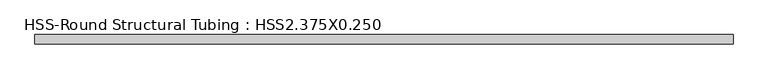
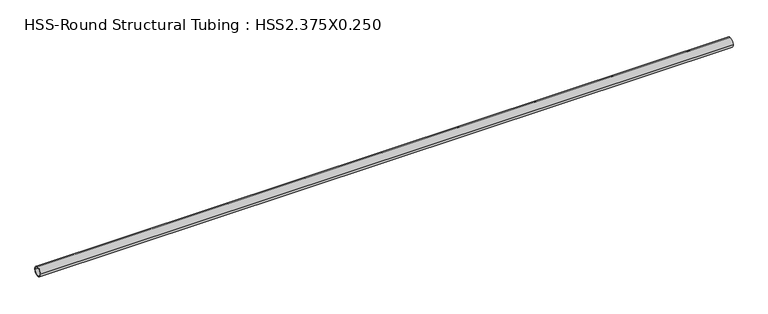
"""IFC4 building model written with IfcOpenShell, lengths in millimetres: beam geometry, HSS-Round Structural Tubing : HSS2.375X0.250."""

from ifc_helpers import new_model, si_unit, point, frame, origin, origin_2d, place, context, project, spatial, circle_curve, trimmed, segment, composite_curve, outline, extrude, source, transform, mapped, element, save


def hss_round_structural_tubing_hss2_375x0_250_6ea9b365(model_context):
    return source(origin(), model_context, "Body", "SweptSolid", [
        extrude(outline(composite_curve([segment(trimmed(circle_curve(origin_2d(), 30.1625), [point((-30.1625, 0.0))], [point((30.1625, 0.0))], False, "CARTESIAN"), True, "CONTINUOUS"), segment(trimmed(circle_curve(origin_2d(), 30.1625), [point((30.1625, 0.0))], [point((-30.1625, 0.0))], False, "CARTESIAN"), True, "CONTINUOUS")], self_intersect=False), holes=[composite_curve([segment(trimmed(circle_curve(origin_2d(), 24.2443), [point((24.2443, 0.0))], [point((-24.2443, 0.0))], True, "CARTESIAN"), True, "CONTINUOUS"), segment(trimmed(circle_curve(origin_2d(), 24.2443), [point((-24.2443, 0.0))], [point((24.2443, 0.0))], True, "CARTESIAN"), True, "CONTINUOUS")], self_intersect=False)]), frame((-2207.2112982, 0.0, 0.0), z_axis=(1.0, 0.0, 0.0), x_axis=(0.0, 1.0, 0.0)), (0.0, 0.0, 1.0), 4401.1362982),
    ])


if __name__ == "__main__":
    model = new_model("IFC4")
    model_context = context("Model", 3, world=origin())
    ifc_project = project(units=[si_unit("LENGTHUNIT", "METRE", prefix="MILLI")], contexts=[model_context])
    site = spatial("IfcSite", under=ifc_project)
    building = spatial("IfcBuilding", under=site)
    placement = place(None, origin())
    hss_round_structural_tubing_hss2_375x0_250_shape = hss_round_structural_tubing_hss2_375x0_250_6ea9b365(model_context)
    element("IfcBeam", 1, ObjectType="HSS-Round Structural Tubing : HSS2.375X0.250", at=placement, inside=building, context=model_context, shape_type="MappedRepresentation", body=[
        mapped(hss_round_structural_tubing_hss2_375x0_250_shape, transform((0.0, 0.0, 0.0), x_axis=(1.0, 0.0, 0.0), y_axis=(0.0, 1.0, 0.0), z_axis=(0.0, 0.0, 1.0))),
    ])
    save(model, "model.ifc")

# Revit data of these elements
# Type "HSS-Round Structural Tubing : HSS2.375X0.250"
#   Assembly Code = "B10"
#   t = 0' - 0.233"
#   W = 5.68
#   Length [instance default] = 5' - 0"
#   OD = 0' - 2 3/8"
#   A = 0.0109028 SF
#   Structural Material [instance default] = Steel ASTM A500, Grade B, Round
# Element 1 (IfcBeam, "HSS-Round Structural Tubing : HSS2.375X0.250")
#   Structural Material = Aluminum
#   Materials on its faces: "Aluminum"
# Materials
#   "Steel ASTM A500, Grade B, Round": class "Metal", colour RGB 199 199 199, transparency 0, Description = "Carbon steel", Cost = 0
#   "Aluminum": class "Metal", colour RGB 247 247 247, transparency 0, Description = "Aluminum 6061", Cost = 0
